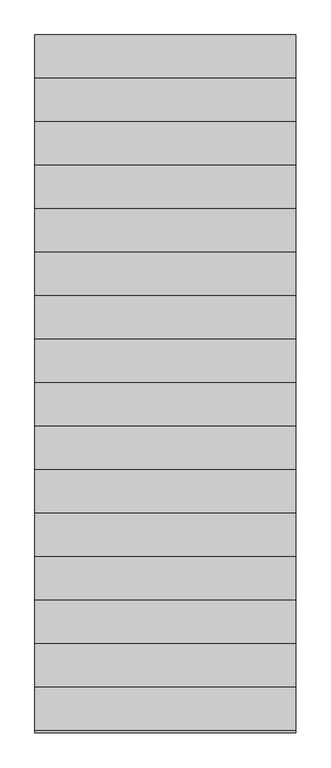
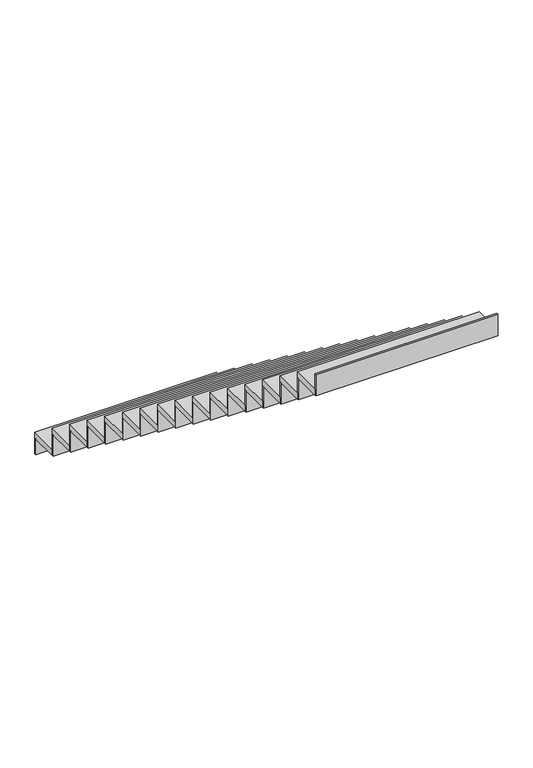
"""IFC4 building model written with IfcOpenShell, lengths in millimetres: stair flight geometry."""

from ifc_helpers import new_model, si_unit, frame, origin, place, context, project, spatial, polyline, outline, extrude, source, transform, mapped, element, save


def stair_flight_c9982ff6(model_context):
    return source(origin(), model_context, "Body", "SweptSolid", [
        extrude(outline(polyline([(-11930.6631644, -7734.8774925), (-11930.6631644, -7722.3774925), (-10430.6631644, -7722.3774925), (-10430.6631644, -7734.8774925), (-11930.6631644, -7734.8774925)])), frame((0.0, 0.0, 2800.0), z_axis=(0.0, 0.0, 1.0), x_axis=(1.0, 0.0, 0.0)), (0.0, 0.0, 1.0), 136.6666667),
        extrude(outline(polyline([(-10430.6631644, -7972.3774925), (-11930.6631644, -7972.3774925), (-11930.6631644, -7722.3774925), (-10430.6631644, -7722.3774925), (-10430.6631644, -7972.3774925)])), frame((0.0, 0.0, 2936.6666667), z_axis=(0.0, 0.0, 1.0), x_axis=(1.0, 0.0, 0.0)), (0.0, 0.0, 1.0), 50.0),
        extrude(outline(polyline([(-11930.6631644, -7984.8774925), (-11930.6631644, -7972.3774925), (-10430.6631644, -7972.3774925), (-10430.6631644, -7984.8774925), (-11930.6631644, -7984.8774925)])), frame((0.0, 0.0, 2936.6666667), z_axis=(0.0, 0.0, 1.0), x_axis=(1.0, 0.0, 0.0)), (0.0, 0.0, 1.0), 186.6666667),
        extrude(outline(polyline([(-10430.6631644, -8222.3774925), (-11930.6631644, -8222.3774925), (-11930.6631644, -7972.3774925), (-10430.6631644, -7972.3774925), (-10430.6631644, -8222.3774925)])), frame((0.0, 0.0, 3123.3333333), z_axis=(0.0, 0.0, 1.0), x_axis=(1.0, 0.0, 0.0)), (0.0, 0.0, 1.0), 50.0),
        extrude(outline(polyline([(-11930.6631644, -8234.8774925), (-11930.6631644, -8222.3774925), (-10430.6631644, -8222.3774925), (-10430.6631644, -8234.8774925), (-11930.6631644, -8234.8774925)])), frame((0.0, 0.0, 3123.3333333), z_axis=(0.0, 0.0, 1.0), x_axis=(1.0, 0.0, 0.0)), (0.0, 0.0, 1.0), 186.6666667),
        extrude(outline(polyline([(-10430.6631644, -8472.3774925), (-11930.6631644, -8472.3774925), (-11930.6631644, -8222.3774925), (-10430.6631644, -8222.3774925), (-10430.6631644, -8472.3774925)])), frame((0.0, 0.0, 3310.0), z_axis=(0.0, 0.0, 1.0), x_axis=(1.0, 0.0, 0.0)), (0.0, 0.0, 1.0), 50.0),
        extrude(outline(polyline([(-11930.6631644, -8484.8774925), (-11930.6631644, -8472.3774925), (-10430.6631644, -8472.3774925), (-10430.6631644, -8484.8774925), (-11930.6631644, -8484.8774925)])), frame((0.0, 0.0, 3310.0), z_axis=(0.0, 0.0, 1.0), x_axis=(1.0, 0.0, 0.0)), (0.0, 0.0, 1.0), 186.6666667),
        extrude(outline(polyline([(-10430.6631644, -8722.3774925), (-11930.6631644, -8722.3774925), (-11930.6631644, -8472.3774925), (-10430.6631644, -8472.3774925), (-10430.6631644, -8722.3774925)])), frame((0.0, 0.0, 3496.6666667), z_axis=(0.0, 0.0, 1.0), x_axis=(1.0, 0.0, 0.0)), (0.0, 0.0, 1.0), 50.0),
        extrude(outline(polyline([(-11930.6631644, -8734.8774925), (-11930.6631644, -8722.3774925), (-10430.6631644, -8722.3774925), (-10430.6631644, -8734.8774925), (-11930.6631644, -8734.8774925)])), frame((0.0, 0.0, 3496.6666667), z_axis=(0.0, 0.0, 1.0), x_axis=(1.0, 0.0, 0.0)), (0.0, 0.0, 1.0), 186.6666667),
        extrude(outline(polyline([(-10430.6631644, -8972.3774925), (-11930.6631644, -8972.3774925), (-11930.6631644, -8722.3774925), (-10430.6631644, -8722.3774925), (-10430.6631644, -8972.3774925)])), frame((0.0, 0.0, 3683.3333333), z_axis=(0.0, 0.0, 1.0), x_axis=(1.0, 0.0, 0.0)), (0.0, 0.0, 1.0), 50.0),
        extrude(outline(polyline([(-11930.6631644, -8984.8774925), (-11930.6631644, -8972.3774925), (-10430.6631644, -8972.3774925), (-10430.6631644, -8984.8774925), (-11930.6631644, -8984.8774925)])), frame((0.0, 0.0, 3683.3333333), z_axis=(0.0, 0.0, 1.0), x_axis=(1.0, 0.0, 0.0)), (0.0, 0.0, 1.0), 186.6666667),
        extrude(outline(polyline([(-10430.6631644, -9222.3774925), (-11930.6631644, -9222.3774925), (-11930.6631644, -8972.3774925), (-10430.6631644, -8972.3774925), (-10430.6631644, -9222.3774925)])), frame((0.0, 0.0, 3870.0), z_axis=(0.0, 0.0, 1.0), x_axis=(1.0, 0.0, 0.0)), (0.0, 0.0, 1.0), 50.0),
        extrude(outline(polyline([(-11930.6631644, -9234.8774925), (-11930.6631644, -9222.3774925), (-10430.6631644, -9222.3774925), (-10430.6631644, -9234.8774925), (-11930.6631644, -9234.8774925)])), frame((0.0, 0.0, 3870.0), z_axis=(0.0, 0.0, 1.0), x_axis=(1.0, 0.0, 0.0)), (0.0, 0.0, 1.0), 186.6666667),
        extrude(outline(polyline([(-10430.6631644, -9472.3774925), (-11930.6631644, -9472.3774925), (-11930.6631644, -9222.3774925), (-10430.6631644, -9222.3774925), (-10430.6631644, -9472.3774925)])), frame((0.0, 0.0, 4056.6666667), z_axis=(0.0, 0.0, 1.0), x_axis=(1.0, 0.0, 0.0)), (0.0, 0.0, 1.0), 50.0),
        extrude(outline(polyline([(-11930.6631644, -9484.8774925), (-11930.6631644, -9472.3774925), (-10430.6631644, -9472.3774925), (-10430.6631644, -9484.8774925), (-11930.6631644, -9484.8774925)])), frame((0.0, 0.0, 4056.6666667), z_axis=(0.0, 0.0, 1.0), x_axis=(1.0, 0.0, 0.0)), (0.0, 0.0, 1.0), 186.6666667),
        extrude(outline(polyline([(-10430.6631644, -9722.3774925), (-11930.6631644, -9722.3774925), (-11930.6631644, -9472.3774925), (-10430.6631644, -9472.3774925), (-10430.6631644, -9722.3774925)])), frame((0.0, 0.0, 4243.3333333), z_axis=(0.0, 0.0, 1.0), x_axis=(1.0, 0.0, 0.0)), (0.0, 0.0, 1.0), 50.0),
        extrude(outline(polyline([(-11930.6631644, -9734.8774925), (-11930.6631644, -9722.3774925), (-10430.6631644, -9722.3774925), (-10430.6631644, -9734.8774925), (-11930.6631644, -9734.8774925)])), frame((0.0, 0.0, 4243.3333333), z_axis=(0.0, 0.0, 1.0), x_axis=(1.0, 0.0, 0.0)), (0.0, 0.0, 1.0), 186.6666667),
        extrude(outline(polyline([(-10430.6631644, -9972.3774925), (-11930.6631644, -9972.3774925), (-11930.6631644, -9722.3774925), (-10430.6631644, -9722.3774925), (-10430.6631644, -9972.3774925)])), frame((0.0, 0.0, 4430.0), z_axis=(0.0, 0.0, 1.0), x_axis=(1.0, 0.0, 0.0)), (0.0, 0.0, 1.0), 50.0),
        extrude(outline(polyline([(-11930.6631644, -9984.8774925), (-11930.6631644, -9972.3774925), (-10430.6631644, -9972.3774925), (-10430.6631644, -9984.8774925), (-11930.6631644, -9984.8774925)])), frame((0.0, 0.0, 4430.0), z_axis=(0.0, 0.0, 1.0), x_axis=(1.0, 0.0, 0.0)), (0.0, 0.0, 1.0), 186.6666667),
        extrude(outline(polyline([(-10430.6631644, -10222.3774925), (-11930.6631644, -10222.3774925), (-11930.6631644, -9972.3774925), (-10430.6631644, -9972.3774925), (-10430.6631644, -10222.3774925)])), frame((0.0, 0.0, 4616.6666667), z_axis=(0.0, 0.0, 1.0), x_axis=(1.0, 0.0, 0.0)), (0.0, 0.0, 1.0), 50.0),
        extrude(outline(polyline([(-11930.6631644, -10234.8774925), (-11930.6631644, -10222.3774925), (-10430.6631644, -10222.3774925), (-10430.6631644, -10234.8774925), (-11930.6631644, -10234.8774925)])), frame((0.0, 0.0, 4616.6666667), z_axis=(0.0, 0.0, 1.0), x_axis=(1.0, 0.0, 0.0)), (0.0, 0.0, 1.0), 186.6666667),
        extrude(outline(polyline([(-10430.6631644, -10472.3774925), (-11930.6631644, -10472.3774925), (-11930.6631644, -10222.3774925), (-10430.6631644, -10222.3774925), (-10430.6631644, -10472.3774925)])), frame((0.0, 0.0, 4803.3333333), z_axis=(0.0, 0.0, 1.0), x_axis=(1.0, 0.0, 0.0)), (0.0, 0.0, 1.0), 50.0),
        extrude(outline(polyline([(-11930.6631644, -10484.8774925), (-11930.6631644, -10472.3774925), (-10430.6631644, -10472.3774925), (-10430.6631644, -10484.8774925), (-11930.6631644, -10484.8774925)])), frame((0.0, 0.0, 4803.3333333), z_axis=(0.0, 0.0, 1.0), x_axis=(1.0, 0.0, 0.0)), (0.0, 0.0, 1.0), 186.6666667),
        extrude(outline(polyline([(-10430.6631644, -10722.3774925), (-11930.6631644, -10722.3774925), (-11930.6631644, -10472.3774925), (-10430.6631644, -10472.3774925), (-10430.6631644, -10722.3774925)])), frame((0.0, 0.0, 4990.0), z_axis=(0.0, 0.0, 1.0), x_axis=(1.0, 0.0, 0.0)), (0.0, 0.0, 1.0), 50.0),
        extrude(outline(polyline([(-11930.6631644, -10734.8774925), (-11930.6631644, -10722.3774925), (-10430.6631644, -10722.3774925), (-10430.6631644, -10734.8774925), (-11930.6631644, -10734.8774925)])), frame((0.0, 0.0, 4990.0), z_axis=(0.0, 0.0, 1.0), x_axis=(1.0, 0.0, 0.0)), (0.0, 0.0, 1.0), 186.6666667),
        extrude(outline(polyline([(-10430.6631644, -10972.3774925), (-11930.6631644, -10972.3774925), (-11930.6631644, -10722.3774925), (-10430.6631644, -10722.3774925), (-10430.6631644, -10972.3774925)])), frame((0.0, 0.0, 5176.6666667), z_axis=(0.0, 0.0, 1.0), x_axis=(1.0, 0.0, 0.0)), (0.0, 0.0, 1.0), 50.0),
        extrude(outline(polyline([(-11930.6631644, -10984.8774925), (-11930.6631644, -10972.3774925), (-10430.6631644, -10972.3774925), (-10430.6631644, -10984.8774925), (-11930.6631644, -10984.8774925)])), frame((0.0, 0.0, 5176.6666667), z_axis=(0.0, 0.0, 1.0), x_axis=(1.0, 0.0, 0.0)), (0.0, 0.0, 1.0), 186.6666667),
        extrude(outline(polyline([(-10430.6631644, -11222.3774925), (-11930.6631644, -11222.3774925), (-11930.6631644, -10972.3774925), (-10430.6631644, -10972.3774925), (-10430.6631644, -11222.3774925)])), frame((0.0, 0.0, 5363.3333333), z_axis=(0.0, 0.0, 1.0), x_axis=(1.0, 0.0, 0.0)), (0.0, 0.0, 1.0), 50.0),
        extrude(outline(polyline([(-11930.6631644, -11234.8774925), (-11930.6631644, -11222.3774925), (-10430.6631644, -11222.3774925), (-10430.6631644, -11234.8774925), (-11930.6631644, -11234.8774925)])), frame((0.0, 0.0, 5363.3333333), z_axis=(0.0, 0.0, 1.0), x_axis=(1.0, 0.0, 0.0)), (0.0, 0.0, 1.0), 186.6666667),
        extrude(outline(polyline([(-10430.6631644, -11472.3774925), (-11930.6631644, -11472.3774925), (-11930.6631644, -11222.3774925), (-10430.6631644, -11222.3774925), (-10430.6631644, -11472.3774925)])), frame((0.0, 0.0, 5550.0), z_axis=(0.0, 0.0, 1.0), x_axis=(1.0, 0.0, 0.0)), (0.0, 0.0, 1.0), 50.0),
        extrude(outline(polyline([(-11930.6631644, -11484.8774925), (-11930.6631644, -11472.3774925), (-10430.6631644, -11472.3774925), (-10430.6631644, -11484.8774925), (-11930.6631644, -11484.8774925)])), frame((0.0, 0.0, 5550.0), z_axis=(0.0, 0.0, 1.0), x_axis=(1.0, 0.0, 0.0)), (0.0, 0.0, 1.0), 186.6666667),
        extrude(outline(polyline([(-10430.6631644, -11722.3774925), (-11930.6631644, -11722.3774925), (-11930.6631644, -11472.3774925), (-10430.6631644, -11472.3774925), (-10430.6631644, -11722.3774925)])), frame((0.0, 0.0, 5736.6666667), z_axis=(0.0, 0.0, 1.0), x_axis=(1.0, 0.0, 0.0)), (0.0, 0.0, 1.0), 50.0),
        extrude(outline(polyline([(-11930.6631644, -11734.8774925), (-11930.6631644, -11722.3774925), (-10430.6631644, -11722.3774925), (-10430.6631644, -11734.8774925), (-11930.6631644, -11734.8774925)])), frame((0.0, 0.0, 5736.6666667), z_axis=(0.0, 0.0, 1.0), x_axis=(1.0, 0.0, 0.0)), (0.0, 0.0, 1.0), 186.6666667),
    ])


if __name__ == "__main__":
    model = new_model("IFC4")
    model_context = context("Model", 3, world=origin())
    ifc_project = project(units=[si_unit("LENGTHUNIT", "METRE", prefix="MILLI")], contexts=[model_context])
    site = spatial("IfcSite", under=ifc_project)
    building = spatial("IfcBuilding", under=site)
    placement = place(None, origin())
    stair_flight_shape = stair_flight_c9982ff6(model_context)
    element("IfcStairFlight", 1, at=placement, inside=building, context=model_context, shape_type="MappedRepresentation", body=[
        mapped(stair_flight_shape, transform((0.0, 0.0, 0.0), x_axis=(1.0, 0.0, 0.0), y_axis=(0.0, 1.0, 0.0), z_axis=(0.0, 0.0, 1.0))),
    ])
    save(model, "model.ifc")
